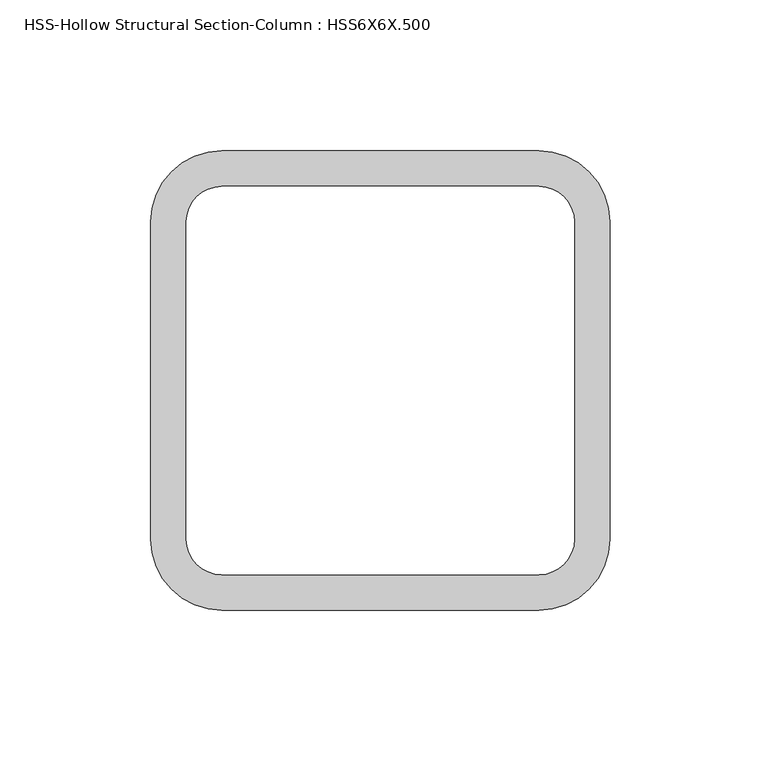
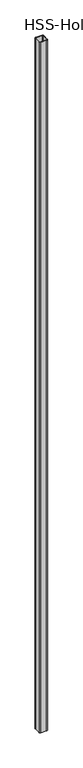
"""IFC4 building model written with IfcOpenShell, lengths in millimetres: column geometry, HSS-Hollow Structural Section-Column : HSS6X6X.500."""

from ifc_helpers import new_model, si_unit, point, frame, frame_2d, origin, place, context, project, spatial, polyline, circle_curve, trimmed, segment, composite_curve, outline, extrude, source, transform, mapped, element, save


def hss_hollow_structural_section_column_hss6x6x_500_d1bc5c07(model_context):
    return source(origin(), model_context, "Body", "SweptSolid", [
        extrude(outline(composite_curve([segment(trimmed(circle_curve(frame_2d((52.5859375, 52.5859375)), 23.6140625), [point((52.5859375, 76.2))], [point((76.2, 52.5859375))], False, "CARTESIAN"), True, "CONTINUOUS"), segment(polyline([(76.2, 52.5859375), (76.2, -52.5859375)]), True, "CONTINUOUS"), segment(trimmed(circle_curve(frame_2d((52.5859375, -52.5859375)), 23.6140625), [point((76.2, -52.5859375))], [point((52.5859375, -76.2))], False, "CARTESIAN"), True, "CONTINUOUS"), segment(polyline([(52.5859375, -76.2), (-52.5859375, -76.2)]), True, "CONTINUOUS"), segment(trimmed(circle_curve(frame_2d((-52.5859375, -52.5859375)), 23.6140625), [point((-52.5859375, -76.2))], [point((-76.2, -52.5859375))], False, "CARTESIAN"), True, "CONTINUOUS"), segment(polyline([(-76.2, -52.5859375), (-76.2, 52.5859375)]), True, "CONTINUOUS"), segment(trimmed(circle_curve(frame_2d((-52.5859375, 52.5859375)), 23.6140625), [point((-76.2, 52.5859375))], [point((-52.5859375, 76.2))], False, "CARTESIAN"), True, "CONTINUOUS"), segment(polyline([(-52.5859375, 76.2), (52.5859375, 76.2)]), True, "CONTINUOUS")], self_intersect=False), holes=[composite_curve([segment(polyline([(52.5859375, 64.3929688), (-52.5859375, 64.3929688)]), True, "CONTINUOUS"), segment(trimmed(circle_curve(frame_2d((-52.5859375, 52.5859375)), 11.8070313), [point((-52.5859375, 64.3929688))], [point((-64.3929688, 52.5859375))], True, "CARTESIAN"), True, "CONTINUOUS"), segment(polyline([(-64.3929688, 52.5859375), (-64.3929688, -52.5859375)]), True, "CONTINUOUS"), segment(trimmed(circle_curve(frame_2d((-52.5859375, -52.5859375)), 11.8070313), [point((-64.3929688, -52.5859375))], [point((-52.5859375, -64.3929687))], True, "CARTESIAN"), True, "CONTINUOUS"), segment(polyline([(-52.5859375, -64.3929687), (52.5859375, -64.3929687)]), True, "CONTINUOUS"), segment(trimmed(circle_curve(frame_2d((52.5859375, -52.5859375)), 11.8070312), [point((52.5859375, -64.3929687))], [point((64.3929687, -52.5859375))], True, "CARTESIAN"), True, "CONTINUOUS"), segment(polyline([(64.3929687, -52.5859375), (64.3929687, 52.5859375)]), True, "CONTINUOUS"), segment(trimmed(circle_curve(frame_2d((52.5859375, 52.5859375)), 11.8070312), [point((64.3929687, 52.5859375))], [point((52.5859375, 64.3929688))], True, "CARTESIAN"), True, "CONTINUOUS")], self_intersect=False)]), frame((0.0, 0.0, -609.6), z_axis=(0.0, 0.0, 1.0), x_axis=(1.0, 0.0, 0.0)), (0.0, 0.0, 1.0), 13157.2),
    ])


if __name__ == "__main__":
    model = new_model("IFC4")
    model_context = context("Model", 3, world=origin())
    ifc_project = project(units=[si_unit("LENGTHUNIT", "METRE", prefix="MILLI")], contexts=[model_context])
    site = spatial("IfcSite", under=ifc_project)
    building = spatial("IfcBuilding", under=site)
    placement = place(None, origin())
    hss_hollow_structural_section_column_hss6x6x_500_shape = hss_hollow_structural_section_column_hss6x6x_500_d1bc5c07(model_context)
    element("IfcColumn", 1, ObjectType="HSS-Hollow Structural Section-Column : HSS6X6X.500", at=placement, inside=building, context=model_context, shape_type="MappedRepresentation", body=[
        mapped(hss_hollow_structural_section_column_hss6x6x_500_shape, transform((0.0, 0.0, 0.0), x_axis=(1.0, 0.0, 0.0), y_axis=(0.0, 1.0, 0.0), z_axis=(0.0, 0.0, 1.0))),
    ])
    save(model, "model.ifc")

# Revit data of these elements
# Type "HSS-Hollow Structural Section-Column : HSS6X6X.500"
#   Assembly Code = "B10"
#   Shape = "Square"
#   W = 35.1
#   Ht = 0' - 6"
#   b = 0' - 6"
#   kr = 0' - 0 119/128"
#   t = 0' - 0 119/256"
#   A = 0.07 SF
#   Structural Material [instance default] = Steel ASTM A500, Grade B, Rectangular and Square
# Element 1 (IfcColumn, "HSS-Hollow Structural Section-Column : HSS6X6X.500")
#   Materials on its faces: "Steel ASTM A500, Grade B, Rectangular and Square"
# Materials
#   "Steel ASTM A500, Grade B, Rectangular and Square": class "Metal", colour RGB 199 199 199, transparency 0, Description = "Carbon steel", Cost = 0
